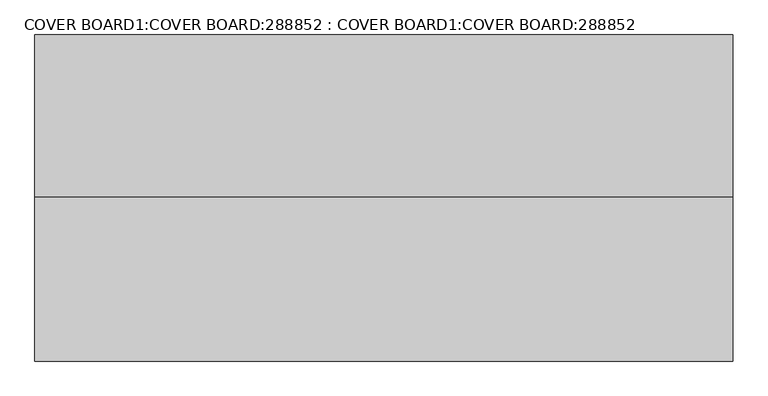
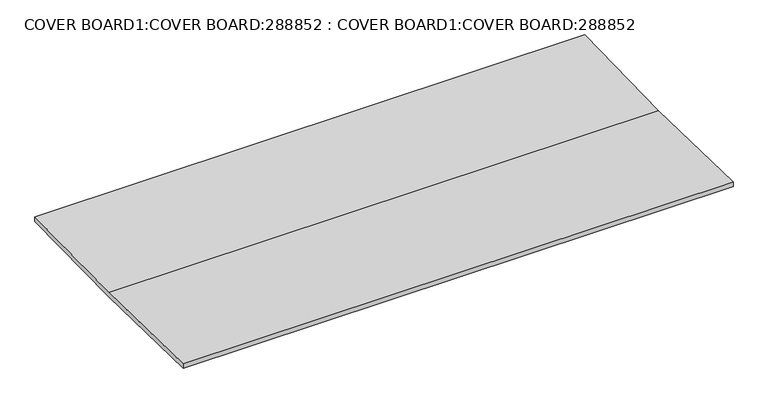
"""IFC4 building model written with IfcOpenShell, lengths in millimetres: proxy geometry, COVER BOARD1:COVER BOARD:288852 : COVER BOARD1:COVER BOARD:288852."""

from ifc_helpers import new_model, si_unit, frame, origin, place, context, project, spatial, polyline, outline, extrude, source, transform, mapped, element, save


def cover_board1_cover_board_288852_cover_board1_cover_board_d5bef7c4(model_context):
    return source(origin(), model_context, "Body", "SweptSolid", [
        extrude(outline(polyline([(-5064.9256348, 40221.0164063), (-4594.6286758, 40211.218553), (-4130.6076102, 40221.0164062), (-4130.6076102, 40203.6846871), (-4594.6286758, 40193.8868338), (-5064.9256348, 40203.6846871), (-5064.9256348, 40221.0164063)])), frame((17159.7769925, 0.0, 0.0), z_axis=(1.0, 0.0, 0.0), x_axis=(0.0, 1.0, 0.0)), (0.0, 0.0, 1.0), 2000.0),
    ])


if __name__ == "__main__":
    model = new_model("IFC4")
    model_context = context("Model", 3, world=origin())
    ifc_project = project(units=[si_unit("LENGTHUNIT", "METRE", prefix="MILLI")], contexts=[model_context])
    site = spatial("IfcSite", under=ifc_project)
    building = spatial("IfcBuilding", under=site)
    placement = place(None, origin())
    cover_board1_cover_board_288852_cover_board1_cover_board_shape = cover_board1_cover_board_288852_cover_board1_cover_board_d5bef7c4(model_context)
    element("IfcBuildingElementProxy", 1, Name="COVER BOARD1:COVER BOARD:288852 : COVER BOARD1:COVER BOARD:288852", ObjectType="COVER BOARD1:COVER BOARD:288852 : COVER BOARD1:COVER BOARD:288852", at=placement, inside=building, context=model_context, shape_type="MappedRepresentation", body=[
        mapped(cover_board1_cover_board_288852_cover_board1_cover_board_shape, transform((0.0, 0.0, 0.0), x_axis=(1.0, 0.0, 0.0), y_axis=(0.0, 1.0, 0.0), z_axis=(0.0, 0.0, 1.0))),
    ])
    save(model, "model.ifc")

# Revit data of these elements
# Type "COVER BOARD1:COVER BOARD:288852 : COVER BOARD1:COVER BOARD:288852"
#   NameOverride = "COVER BOARD1:COVER BOARD:288852"
#   ObjectTypeOverride = "COVER BOARD1:COVER BOARD"
#   Reference = "COVER BOARD"
#   Category = "Generic Models"
#   Tag = "288852"
# Element 1 (IfcBuildingElementProxy, "COVER BOARD1:COVER BOARD:288852 : COVER BOARD1:COVER BOARD:288852")
#   Materials on its faces: "CDX PLYWOOD - SEE STRUCTURAL DWGS"
# Materials
#   "CDX PLYWOOD - SEE STRUCTURAL DWGS": class "Unassigned", colour RGB 202 163 108, transparency 0, Cost = 0
